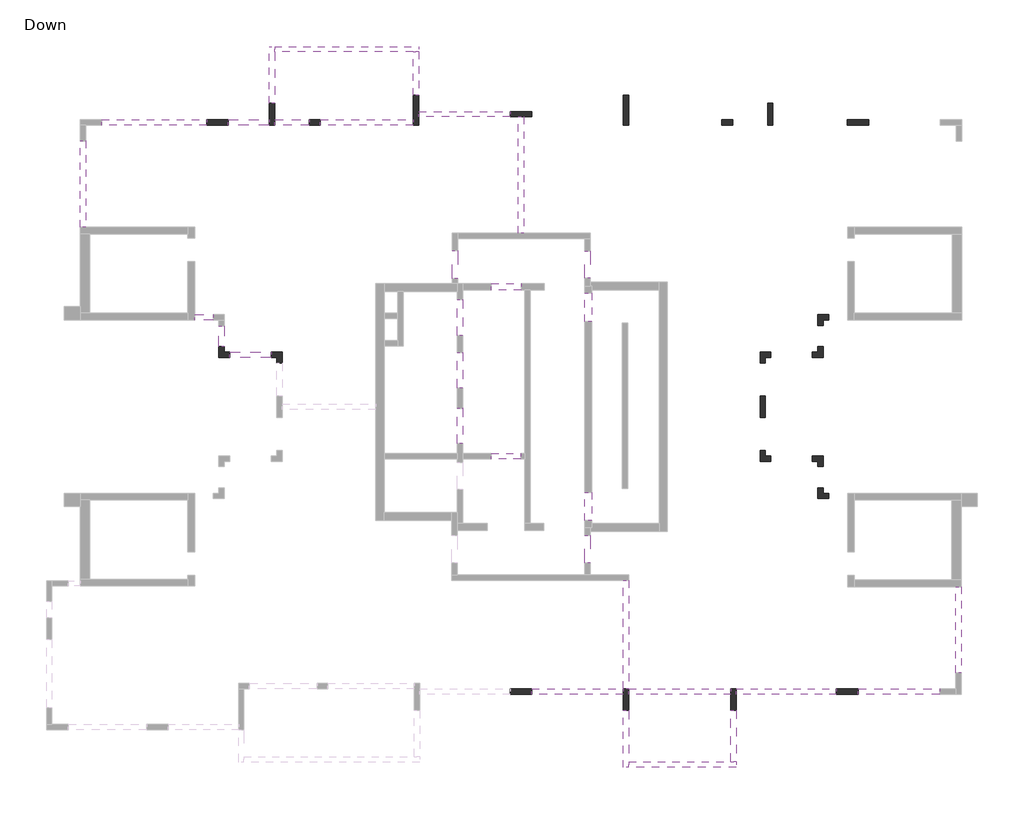
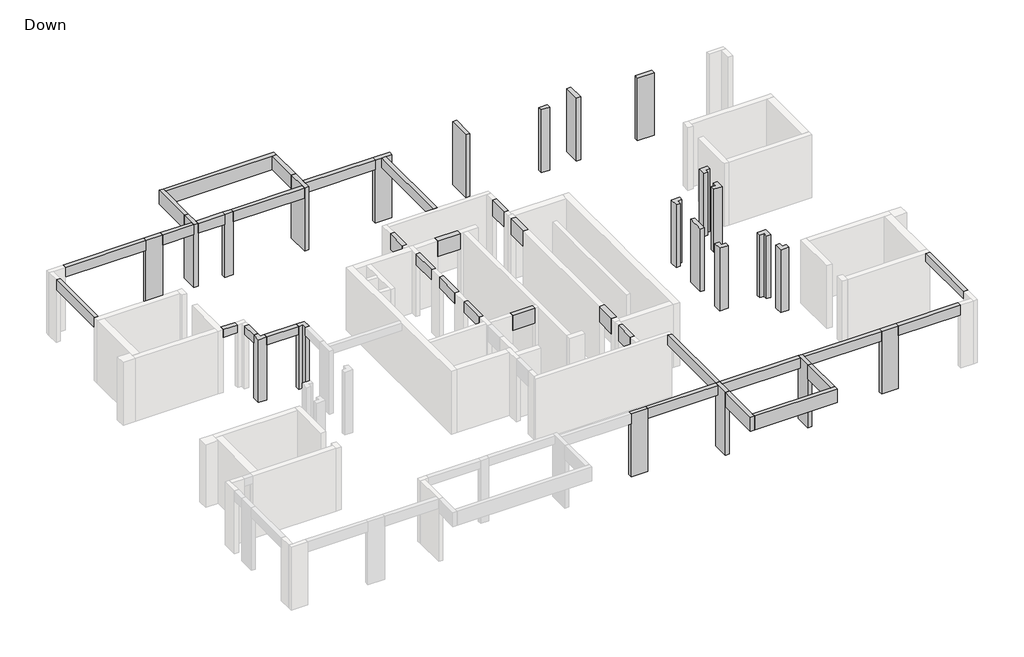
# One storey, part 3 of 3: 32 beams, 22 columns.
# Revit data of these elements (continued)
# Element 46 (IfcColumn, "Concrete Rectengular Column : 20/80") (continued)
#   SOFiSTiK_AMG_Adjusted = yes
#   Structural Material = Concrete
#   Phase Created = New Construction
#   Materials on its faces: "Concrete"
# Element 47 (IfcColumn, "L Column : 40/40/20/20")
#   Comments = ""
#   Mark = "C20"
#   SOFiSTiK_AMG_Comments = ""
#   SOFiSTiK_AMG_Scheduled = yes
#   SOFiSTiK_AMG_Adjusted = yes
#   Structural Material = Concrete
#   Phase Created = New Construction
# Element 48 (IfcColumn, "L Column : 40/40/20/20")
#   Comments = ""
#   Mark = "C21"
#   SOFiSTiK_AMG_Comments = ""
#   SOFiSTiK_AMG_Scheduled = yes
#   SOFiSTiK_AMG_Adjusted = yes
#   Structural Material = Concrete
#   Phase Created = New Construction
# Element 49 (IfcColumn, "L Column : 40/40/20/20")
#   Comments = ""
#   Mark = "C25"
#   SOFiSTiK_AMG_Comments = ""
#   SOFiSTiK_AMG_Scheduled = yes
#   SOFiSTiK_AMG_Adjusted = yes
#   Structural Material = Concrete
#   Phase Created = New Construction
# Element 50 (IfcColumn, "L Column : 40/40/20/20")
#   Comments = ""
#   Mark = "C26"
#   SOFiSTiK_AMG_Comments = ""
#   SOFiSTiK_AMG_Scheduled = yes
#   SOFiSTiK_AMG_Adjusted = yes
#   Structural Material = Concrete
#   Phase Created = New Construction
# Element 51 (IfcColumn, "L Column : 40/40/20/20")
#   Comments = ""
#   Mark = "C27"
#   SOFiSTiK_AMG_Comments = ""
#   SOFiSTiK_AMG_Scheduled = yes
#   SOFiSTiK_AMG_Adjusted = yes
#   Structural Material = Concrete
#   Phase Created = New Construction
# Element 52 (IfcColumn, "L Column : 40/40/20/20")
#   Comments = ""
#   Mark = "C28"
#   SOFiSTiK_AMG_Comments = ""
#   SOFiSTiK_AMG_Scheduled = yes
#   SOFiSTiK_AMG_Adjusted = yes
#   Structural Material = Concrete
#   Phase Created = New Construction
# Element 53 (IfcColumn, "L Column : 40/40/20/20")
#   Comments = ""
#   Mark = "C29"
#   SOFiSTiK_AMG_Comments = ""
#   SOFiSTiK_AMG_Scheduled = yes
#   SOFiSTiK_AMG_Adjusted = yes
#   Structural Material = Concrete
#   Phase Created = New Construction
# Element 54 (IfcColumn, "L Column : 40/40/20/20")
#   Comments = ""
#   Mark = "C30"
#   SOFiSTiK_AMG_Comments = ""
#   SOFiSTiK_AMG_Scheduled = yes
#   SOFiSTiK_AMG_Adjusted = yes
#   Structural Material = Concrete
#   Phase Created = New Construction
# Materials
#   "Concrete": class "Concrete", colour RGB 192 192 192, transparency 0, Keynote = "01000", Description = "Cast-in-place concrete", Cost = 0
#   "Concrete, Cast-in-Place gray": class "Concrete", colour RGB 192 192 192, transparency 0, Description = "Cast-in-place concrete", Cost = 0
